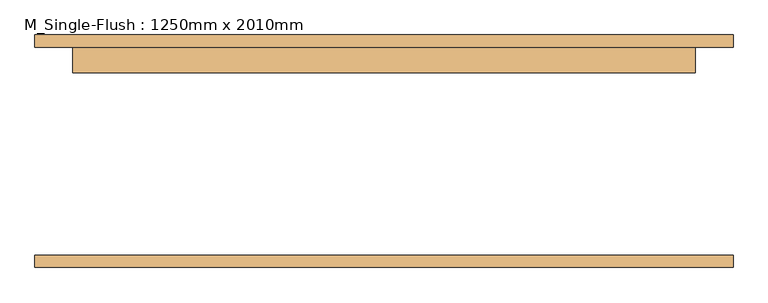
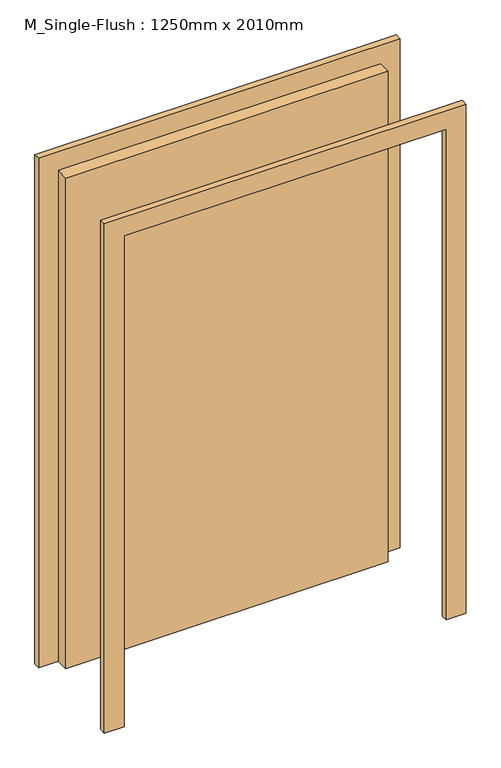
"""IFC4 building model written with IfcOpenShell, lengths in millimetres: door geometry, M_Single-Flush : 1250mm x 2010mm."""

import ifcopenshell
import ifcopenshell.guid

model = None  # the IFC model being written
_history = None  # IfcOwnerHistory: only IFC2X3 demands one
_inside = {}  # id of a spatial element -> (the spatial element, [elements in it])
_under = {}  # id of a project, library or spatial element -> (it, [spatial elements below it])
_declared = {}  # id of a project -> (the project, [libraries it declares])
_typed = {}  # id of a type object -> (the type object, [elements of that type])
_made_of = {}  # id of a material, layer set ... -> (it, [elements and type objects made of it])


def new_model(schema):
    """Start an empty IFC model of exactly this schema.

    Asked for "IFC4X3", IfcOpenShell would pick the latest addendum, in which some entities
    have other attributes; the version numbers below select the first issue.
    IFC2X3 requires an IfcOwnerHistory on every rooted entity: one is made here for all.
    """
    global model, _history
    if schema == "IFC4X3":
        model = ifcopenshell.file(schema_version=(4, 3, 0, 0))
    else:
        model = ifcopenshell.file(schema=schema)
    _inside.clear()
    _under.clear()
    _declared.clear()
    _typed.clear()
    _made_of.clear()
    _history = None
    if model.schema == "IFC2X3":
        org = make("IfcOrganization", Name="unknown")
        user = make(
            "IfcPersonAndOrganization",
            ThePerson=make("IfcPerson", FamilyName="unknown"),
            TheOrganization=org,
        )
        app = make(
            "IfcApplication",
            ApplicationDeveloper=org,
            Version="unknown",
            ApplicationFullName="unknown",
            ApplicationIdentifier="unknown",
        )
        _history = make(
            "IfcOwnerHistory",
            OwningUser=user,
            OwningApplication=app,
            ChangeAction="ADDED",
            CreationDate=0,
        )
    return model


def make(cls, **values):
    """One entity of the class cls with the attributes given. An attribute that is None is left unset."""
    return model.create_entity(
        cls, **{name: value for name, value in values.items() if value is not None}
    )


def rooted(cls, **values):
    """An entity with a GlobalId (a new one), such as an element, a storey or a relation."""
    return make(cls, GlobalId=ifcopenshell.guid.new(), OwnerHistory=_history, **values)


def si_unit(unit_type, name, prefix=None):
    """IfcSIUnit, for example si_unit("LENGTHUNIT", "METRE", prefix="MILLI")."""
    return make("IfcSIUnit", UnitType=unit_type, Prefix=prefix, Name=name)


def assignment(units):
    """IfcUnitAssignment: the units of a project."""
    return None if units is None else make("IfcUnitAssignment", Units=units)


def point(xyz):
    """IfcCartesianPoint."""
    return None if xyz is None else make("IfcCartesianPoint", Coordinates=xyz)


def direction(xyz):
    """IfcDirection."""
    return None if xyz is None else make("IfcDirection", DirectionRatios=xyz)


def frame(location, z_axis=None, x_axis=None):
    """IfcAxis2Placement3D, a coordinate frame: its origin and axes. An axis left out is left unset."""
    return make(
        "IfcAxis2Placement3D",
        Location=point(location),
        Axis=direction(z_axis),
        RefDirection=direction(x_axis),
    )


def origin():
    """The frame at (0, 0, 0) with its axes left unset."""
    return frame((0.0, 0.0, 0.0))


def origin_with_axes():
    """The frame at (0, 0, 0) with the z axis (0, 0, 1) and the x axis (1, 0, 0) written out."""
    return frame((0.0, 0.0, 0.0), z_axis=(0.0, 0.0, 1.0), x_axis=(1.0, 0.0, 0.0))


def place(relative_to, where):
    """IfcLocalPlacement: puts the frame where relative to a parent placement (None: the world)."""
    return make(
        "IfcLocalPlacement", PlacementRelTo=relative_to, RelativePlacement=where
    )


def context(
    kind, dimensions, precision=None, world=None, true_north=None, identifier=None
):
    """IfcGeometricRepresentationContext, for example the 3D "Model" context."""
    return make(
        "IfcGeometricRepresentationContext",
        ContextIdentifier=identifier,
        ContextType=kind,
        CoordinateSpaceDimension=dimensions,
        Precision=precision,
        WorldCoordinateSystem=world,
        TrueNorth=true_north,
    )


def project(units=None, contexts=None):
    """IfcProject with its units and contexts."""
    return rooted(
        "IfcProject",
        Name="project",
        RepresentationContexts=contexts,
        UnitsInContext=assignment(units),
    )


def spatial(cls, under=None, at=None, **own):
    """A site, building, storey or space (cls), placed at a placement, below another one or the project."""
    s = rooted(cls, ObjectPlacement=at, **own)
    if under is not None:
        _under.setdefault(under.id(), (under, []))[1].append(s)
    return s


def polyline(points):
    """IfcPolyline through the points."""
    return make("IfcPolyline", Points=[point(p) for p in points])


def outline(outer, holes=None, kind="AREA"):
    """IfcArbitraryClosedProfileDef: a profile drawn as a closed curve; with holes, ...WithVoids."""
    if holes is None:
        return make("IfcArbitraryClosedProfileDef", ProfileType=kind, OuterCurve=outer)
    return make(
        "IfcArbitraryProfileDefWithVoids",
        ProfileType=kind,
        OuterCurve=outer,
        InnerCurves=holes,
    )


def extrude(swept, where, along, depth):
    """IfcExtrudedAreaSolid: the profile swept, set in the frame where, extruded along a direction by depth."""
    return make(
        "IfcExtrudedAreaSolid",
        SweptArea=swept,
        Position=where,
        ExtrudedDirection=direction(along),
        Depth=depth,
    )


def shape(context_of_items, identifier, shape_type, items):
    """IfcShapeRepresentation: the items that make up one representation, for example the "Body"."""
    return make(
        "IfcShapeRepresentation",
        ContextOfItems=context_of_items,
        RepresentationIdentifier=identifier,
        RepresentationType=shape_type,
        Items=items,
    )


def source(mapping_origin, context_of_items, identifier, shape_type, items):
    """IfcRepresentationMap: a shape defined once, which mapped items show again and again."""
    return make(
        "IfcRepresentationMap",
        MappingOrigin=mapping_origin,
        MappedRepresentation=shape(context_of_items, identifier, shape_type, items),
    )


def transform(
    local_origin,
    x_axis=None,
    y_axis=None,
    z_axis=None,
    scale=None,
    scale2=None,
    scale3=None,
    uniform=True,
):
    """IfcCartesianTransformationOperator3D, or its non-uniform kind. x_axis, y_axis, z_axis: its Axis1, 2, 3."""
    if uniform:
        return make(
            "IfcCartesianTransformationOperator3D",
            Axis1=direction(x_axis),
            Axis2=direction(y_axis),
            LocalOrigin=point(local_origin),
            Scale=scale,
            Axis3=direction(z_axis),
        )
    return make(
        "IfcCartesianTransformationOperator3DnonUniform",
        Axis1=direction(x_axis),
        Axis2=direction(y_axis),
        LocalOrigin=point(local_origin),
        Scale=scale,
        Axis3=direction(z_axis),
        Scale2=scale2,
        Scale3=scale3,
    )


def mapped(mapping_source, mapping_target):
    """IfcMappedItem: shows the shape of a source again, moved by a transform."""
    return make(
        "IfcMappedItem", MappingSource=mapping_source, MappingTarget=mapping_target
    )


def made_of(thing, what):
    """Note that an element or type object is made of a material, layer set ...; save() writes the relation."""
    if what is not None:
        _made_of.setdefault(what.id(), (what, []))[1].append(thing)
    return thing


def element(
    cls,
    number,
    at=None,
    inside=None,
    cuts=None,
    type_object=None,
    material=None,
    context=None,
    identifier="Body",
    shape_type=None,
    held_by="IfcProductDefinitionShape",
    body=None,
    shapes=None,
    **own,
):
    """One element of the class cls, such as IfcWall. Its Tag is "e" and its number.

    at: its placement. inside: the storey or other place that contains it. cuts: it is an
    opening in that element (IfcRelVoidsElement). A single representation is given by context,
    identifier, shape_type and body (its items); several are given by shapes. held_by: the class
    of the entity that holds the representations. save() writes the other relations.
    """
    e = rooted(cls, Tag="e%d" % number, ObjectPlacement=at, **own)
    if body is not None:
        shapes = [shape(context, identifier, shape_type, body)]
    if shapes is not None:
        e.Representation = make(held_by, Representations=shapes)
    if inside is not None:
        _inside.setdefault(inside.id(), (inside, []))[1].append(e)
    if cuts is not None:
        rooted(
            "IfcRelVoidsElement", RelatingBuildingElement=cuts, RelatedOpeningElement=e
        )
    if type_object is not None:
        _typed.setdefault(type_object.id(), (type_object, []))[1].append(e)
    return made_of(e, material)


def aggregate(whole, parts):
    """IfcRelAggregates: a whole, such as a stair, and the parts it consists of."""
    return rooted("IfcRelAggregates", RelatingObject=whole, RelatedObjects=parts)


def save(model, path):
    """Write the relations noted so far, then the file.

    IfcRelAggregates (storeys below a building ...), IfcRelContainedInSpatialStructure (elements
    in a storey), IfcRelDefinesByType, IfcRelAssociatesMaterial and IfcRelDeclares: one each for
    every whole, place, type object, material and project.
    """
    for whole, parts in _under.values():
        aggregate(whole, parts)
    for where, things in _inside.values():
        rooted(
            "IfcRelContainedInSpatialStructure",
            RelatedElements=things,
            RelatingStructure=where,
        )
    for kind, things in _typed.values():
        rooted("IfcRelDefinesByType", RelatedObjects=things, RelatingType=kind)
    for what, things in _made_of.values():
        rooted("IfcRelAssociatesMaterial", RelatedObjects=things, RelatingMaterial=what)
    for by, libraries in _declared.values():
        rooted("IfcRelDeclares", RelatingContext=by, RelatedDefinitions=libraries)
    model.write(path)


def m_single_flush_1250mm_x_2010mm_0100e384(model_context):
    return source(origin(), model_context, "Body", "SweptSolid", [
        extrude(outline(polyline([(2086.0, -701.0), (0.0, -701.0), (0.0, -625.0), (2010.0, -625.0), (2010.0, 625.0), (0.0, 625.0), (0.0, 701.0), (2086.0, 701.0), (2086.0, -701.0)])), frame((0.0, 208.5, 0.0), z_axis=(0.0, 1.0, 0.0), x_axis=(0.0, 0.0, 1.0)), (0.0, 0.0, 1.0), 25.0),
        extrude(outline(polyline([(2086.0, 701.0), (2086.0, -701.0), (0.0, -701.0), (0.0, -625.0), (2010.0, -625.0), (2010.0, 625.0), (0.0, 625.0), (0.0, 701.0), (2086.0, 701.0)])), frame((0.0, -233.5, 0.0), z_axis=(0.0, 1.0, 0.0), x_axis=(0.0, 0.0, 1.0)), (0.0, 0.0, 1.0), 25.0),
        extrude(outline(polyline([(625.0, 157.5), (-625.0, 157.5), (-625.0, 208.5), (625.0, 208.5), (625.0, 157.5)])), origin_with_axes(), (0.0, 0.0, 1.0), 2010.0),
    ])


if __name__ == "__main__":
    model = new_model("IFC4")
    model_context = context("Model", 3, world=origin())
    ifc_project = project(units=[si_unit("LENGTHUNIT", "METRE", prefix="MILLI")], contexts=[model_context])
    site = spatial("IfcSite", under=ifc_project)
    building = spatial("IfcBuilding", under=site)
    placement = place(None, origin())
    m_single_flush_1250mm_x_2010mm_shape = m_single_flush_1250mm_x_2010mm_0100e384(model_context)
    element("IfcDoor", 1, ObjectType="M_Single-Flush : 1250mm x 2010mm", at=placement, inside=building, context=model_context, shape_type="MappedRepresentation", body=[
        mapped(m_single_flush_1250mm_x_2010mm_shape, transform((0.0, 0.0, 0.0), x_axis=(1.0, 0.0, 0.0), y_axis=(0.0, 1.0, 0.0), z_axis=(0.0, 0.0, 1.0))),
    ])
    save(model, "model.ifc")

# Revit data of these elements
# Project information
#   Host = "https://172.16.10.122:8080/projects"
#   Project Issue Date = "Issue Date"
#   Project Status = "Project Status"
#   Client Name = "Owner"
#   Project Address = "Enter address here"
#   Project Name = "Duplex Apartment"
#   Project Number = "1001"
#   Category Description = "Duplex"
#   Category Code = "11-16 21 11"
# Type "M_Single-Flush : 1250mm x 2010mm"
#   Manufacturer = "Manufacturer"
#   Type Mark = "33"
#   Construction Type = "Construction Type"
#   Fire Rating = "Fire Rating"
#   AccessibilityPerformance = "AccessibilityPerformance"
#   CodePerformance = "CodePerformance"
#   IsFireExit = "IsFireExit"
#   ConstructionType = "ConstructionType"
#   GlazingAreaFraction = "GlazingAreaFraction"
#   OperationType = "OperationType"
#   Area = "Area"
#   Color = "Color"
#   Constituents = "Constituents"
#   Features = "Features"
#   Finish = "Finish"
#   Grade = "Grade"
#   Material = "Material"
#   ModelReference = "ModelReference"
#   NominalHeight = "NominalHeight"
#   NominalLength = "NominalLength"
#   NominalWidth = "NominalWidth"
#   ProductionYear = "ProductionYear"
#   Reference = "Reference"
#   Shape = "Shape"
#   Size = "Size"
#   SustainabilityPerformance = "SustainabilityPerformance"
#   WarrantyDescription = "WarrantyDescription"
#   WarrantyDurationLabor = "WarrantyDurationLabor"
#   WarrantyDurationParts = "WarrantyDurationParts"
#   WarrantyGuarantorLabor = "WarrantyGuarantorLabor"
#   WarrantyGuarantorParts = "WarrantyGuarantorParts"
#   ExpectedLife = "ExpectedLife"
#   ReplacementCost = "ReplacementCost"
#   AssetAccountingType = "FIXED"
#   ModelLabel = "ModelLabel"
#   Thickness = 0.051 m
#   Height = 2.010 m
#   Trim Projection Ext = 0.025 m
#   Trim Projection Int = 0.025 m
#   Trim Width = 0.076 m
#   Width = 1.250 m
#   Function = 1
#   Door Material = Door - Panel
#   Frame Material = Door - Frame
#   Wall Closure = (empty or 0)
# Element 1 (IfcDoor, "M_Single-Flush : 1250mm x 2010mm")
#   Materials on its faces: "Door - Frame", "Door - Panel"
# Materials
#   "Door - Panel": class "Wood", colour RGB 210 159 95, transparency 0
#   "Door - Frame": class "Miscellaneous", colour RGB 118 70 51, transparency 0
